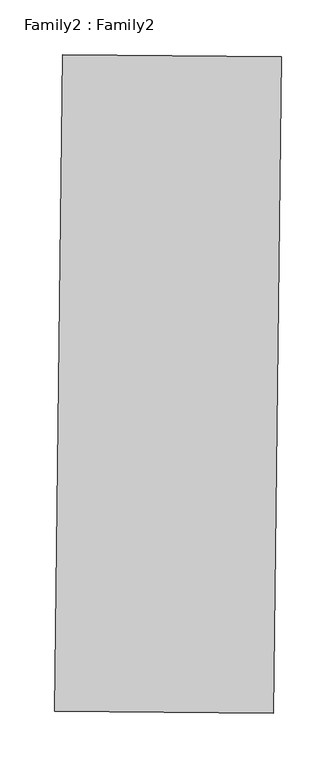
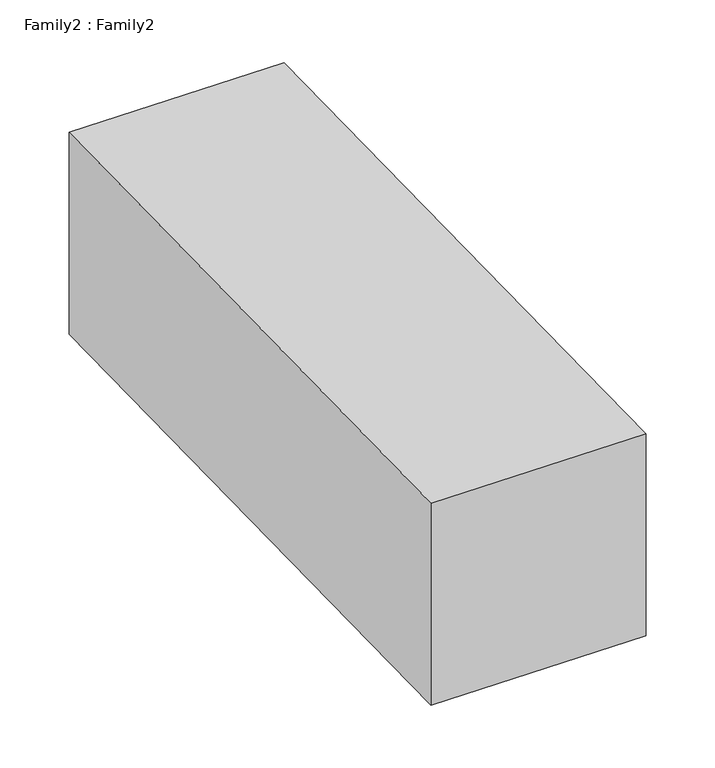
"""IFC4 building model written with IfcOpenShell, lengths in millimetres: proxy geometry, Family2 : Family2."""

from ifc_helpers import new_model, si_unit, origin, place, context, project, spatial, faceted_brep, source, transform, mapped, element, save


def family2_family2_4fb73a58(model_context):
    return source(origin(), model_context, "Body", "Brep", [
        faceted_brep([(-3947.0499544, -6373.591465, 1.0945136), (-3947.0499544, -6373.591465, 201.0945136), (-3939.7928401, -5774.0086576, 202.060409), (-3939.7928401, -5774.0086576, 2.060409), (-3747.0587644, -6375.4686776, 201.0945136), (-3739.8016501, -5775.8858703, 202.060409), (-3747.0587644, -6375.4686776, 1.0945136), (-3739.8016501, -5775.8858703, 2.060409)], [[[0, 1, 2, 3]], [[1, 4, 5, 2]], [[4, 6, 7, 5]], [[6, 0, 3, 7]], [[3, 2, 5, 7]], [[0, 6, 4, 1]]]),
    ])


if __name__ == "__main__":
    model = new_model("IFC4")
    model_context = context("Model", 3, world=origin())
    ifc_project = project(units=[si_unit("LENGTHUNIT", "METRE", prefix="MILLI")], contexts=[model_context])
    site = spatial("IfcSite", under=ifc_project)
    building = spatial("IfcBuilding", under=site)
    placement = place(None, origin())
    family2_family2_shape = family2_family2_4fb73a58(model_context)
    element("IfcBuildingElementProxy", 1, Name="Family2 : Family2", ObjectType="Family2 : Family2", at=placement, inside=building, context=model_context, shape_type="MappedRepresentation", body=[
        mapped(family2_family2_shape, transform((0.0, 0.0, 0.0), x_axis=(1.0, 0.0, 0.0), y_axis=(0.0, 1.0, 0.0), z_axis=(0.0, 0.0, 1.0))),
    ])
    save(model, "model.ifc")

# Revit data of these elements
# Type "Family2 : Family2"
#   Default Elevation = 0
